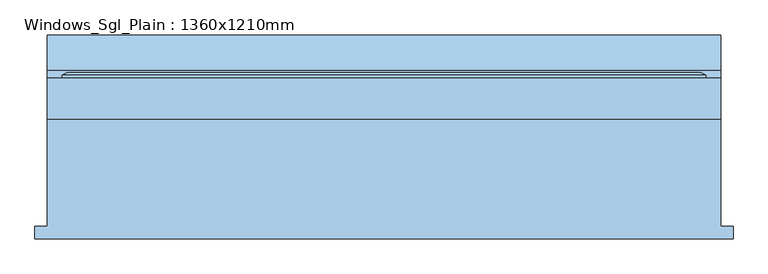
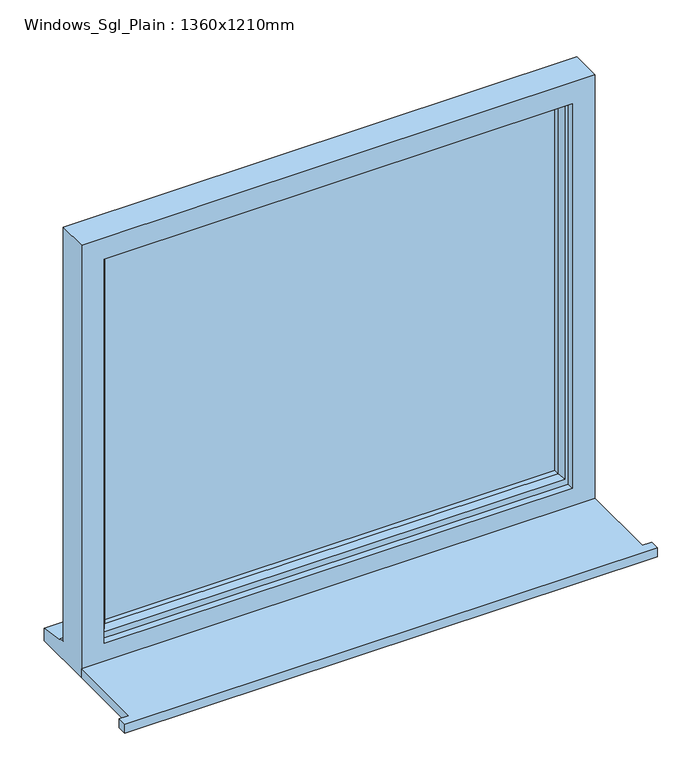
"""IFC4 building model written with IfcOpenShell, lengths in millimetres: window geometry, Windows_Sgl_Plain : 1360x1210mm."""

import ifcopenshell
import ifcopenshell.guid

model = None  # the IFC model being written
_history = None  # IfcOwnerHistory: only IFC2X3 demands one
_inside = {}  # id of a spatial element -> (the spatial element, [elements in it])
_under = {}  # id of a project, library or spatial element -> (it, [spatial elements below it])
_declared = {}  # id of a project -> (the project, [libraries it declares])
_typed = {}  # id of a type object -> (the type object, [elements of that type])
_made_of = {}  # id of a material, layer set ... -> (it, [elements and type objects made of it])


def new_model(schema):
    """Start an empty IFC model of exactly this schema.

    Asked for "IFC4X3", IfcOpenShell would pick the latest addendum, in which some entities
    have other attributes; the version numbers below select the first issue.
    IFC2X3 requires an IfcOwnerHistory on every rooted entity: one is made here for all.
    """
    global model, _history
    if schema == "IFC4X3":
        model = ifcopenshell.file(schema_version=(4, 3, 0, 0))
    else:
        model = ifcopenshell.file(schema=schema)
    _inside.clear()
    _under.clear()
    _declared.clear()
    _typed.clear()
    _made_of.clear()
    _history = None
    if model.schema == "IFC2X3":
        org = make("IfcOrganization", Name="unknown")
        user = make(
            "IfcPersonAndOrganization",
            ThePerson=make("IfcPerson", FamilyName="unknown"),
            TheOrganization=org,
        )
        app = make(
            "IfcApplication",
            ApplicationDeveloper=org,
            Version="unknown",
            ApplicationFullName="unknown",
            ApplicationIdentifier="unknown",
        )
        _history = make(
            "IfcOwnerHistory",
            OwningUser=user,
            OwningApplication=app,
            ChangeAction="ADDED",
            CreationDate=0,
        )
    return model


def make(cls, **values):
    """One entity of the class cls with the attributes given. An attribute that is None is left unset."""
    return model.create_entity(
        cls, **{name: value for name, value in values.items() if value is not None}
    )


def rooted(cls, **values):
    """An entity with a GlobalId (a new one), such as an element, a storey or a relation."""
    return make(cls, GlobalId=ifcopenshell.guid.new(), OwnerHistory=_history, **values)


def si_unit(unit_type, name, prefix=None):
    """IfcSIUnit, for example si_unit("LENGTHUNIT", "METRE", prefix="MILLI")."""
    return make("IfcSIUnit", UnitType=unit_type, Prefix=prefix, Name=name)


def assignment(units):
    """IfcUnitAssignment: the units of a project."""
    return None if units is None else make("IfcUnitAssignment", Units=units)


def point(xyz):
    """IfcCartesianPoint."""
    return None if xyz is None else make("IfcCartesianPoint", Coordinates=xyz)


def direction(xyz):
    """IfcDirection."""
    return None if xyz is None else make("IfcDirection", DirectionRatios=xyz)


def frame(location, z_axis=None, x_axis=None):
    """IfcAxis2Placement3D, a coordinate frame: its origin and axes. An axis left out is left unset."""
    return make(
        "IfcAxis2Placement3D",
        Location=point(location),
        Axis=direction(z_axis),
        RefDirection=direction(x_axis),
    )


def origin():
    """The frame at (0, 0, 0) with its axes left unset."""
    return frame((0.0, 0.0, 0.0))


def place(relative_to, where):
    """IfcLocalPlacement: puts the frame where relative to a parent placement (None: the world)."""
    return make(
        "IfcLocalPlacement", PlacementRelTo=relative_to, RelativePlacement=where
    )


def context(
    kind, dimensions, precision=None, world=None, true_north=None, identifier=None
):
    """IfcGeometricRepresentationContext, for example the 3D "Model" context."""
    return make(
        "IfcGeometricRepresentationContext",
        ContextIdentifier=identifier,
        ContextType=kind,
        CoordinateSpaceDimension=dimensions,
        Precision=precision,
        WorldCoordinateSystem=world,
        TrueNorth=true_north,
    )


def project(units=None, contexts=None):
    """IfcProject with its units and contexts."""
    return rooted(
        "IfcProject",
        Name="project",
        RepresentationContexts=contexts,
        UnitsInContext=assignment(units),
    )


def spatial(cls, under=None, at=None, **own):
    """A site, building, storey or space (cls), placed at a placement, below another one or the project."""
    s = rooted(cls, ObjectPlacement=at, **own)
    if under is not None:
        _under.setdefault(under.id(), (under, []))[1].append(s)
    return s


def polyline(points):
    """IfcPolyline through the points."""
    return make("IfcPolyline", Points=[point(p) for p in points])


def outline(outer, holes=None, kind="AREA"):
    """IfcArbitraryClosedProfileDef: a profile drawn as a closed curve; with holes, ...WithVoids."""
    if holes is None:
        return make("IfcArbitraryClosedProfileDef", ProfileType=kind, OuterCurve=outer)
    return make(
        "IfcArbitraryProfileDefWithVoids",
        ProfileType=kind,
        OuterCurve=outer,
        InnerCurves=holes,
    )


def extrude(swept, where, along, depth):
    """IfcExtrudedAreaSolid: the profile swept, set in the frame where, extruded along a direction by depth."""
    return make(
        "IfcExtrudedAreaSolid",
        SweptArea=swept,
        Position=where,
        ExtrudedDirection=direction(along),
        Depth=depth,
    )


def faces_of(points, faces, orient=None, outer=None):
    """IfcFace entities. A face is a list of loops; a loop is a list of indices into points, from 0.

    orient and outer hold one flag for each loop. By default every Orientation is true, the
    first loop of a face is its IfcFaceOuterBound and the others are IfcFaceBound.
    """
    made = []
    for i, loops in enumerate(faces):
        bounds = []
        for j, loop in enumerate(loops):
            is_outer = j == 0 if outer is None else outer[i][j]
            bounds.append(
                make(
                    "IfcFaceOuterBound" if is_outer else "IfcFaceBound",
                    Bound=make("IfcPolyLoop", Polygon=[points[k] for k in loop]),
                    Orientation=True if orient is None else orient[i][j],
                )
            )
        made.append(make("IfcFace", Bounds=bounds))
    return made


def faceted_brep(points, faces, orient=None, outer=None, voids=None):
    """IfcFacetedBrep: a solid bounded by flat faces; with voids (closed shells), ...WithVoids."""
    shared = [point(p) for p in points]
    hull = make("IfcClosedShell", CfsFaces=faces_of(shared, faces, orient, outer))
    if voids is None:
        return make("IfcFacetedBrep", Outer=hull)
    return make(
        "IfcFacetedBrepWithVoids",
        Outer=hull,
        Voids=[
            make(cls, CfsFaces=faces_of(shared, fs, o, b)) for cls, fs, o, b in voids
        ],
    )


def shape(context_of_items, identifier, shape_type, items):
    """IfcShapeRepresentation: the items that make up one representation, for example the "Body"."""
    return make(
        "IfcShapeRepresentation",
        ContextOfItems=context_of_items,
        RepresentationIdentifier=identifier,
        RepresentationType=shape_type,
        Items=items,
    )


def source(mapping_origin, context_of_items, identifier, shape_type, items):
    """IfcRepresentationMap: a shape defined once, which mapped items show again and again."""
    return make(
        "IfcRepresentationMap",
        MappingOrigin=mapping_origin,
        MappedRepresentation=shape(context_of_items, identifier, shape_type, items),
    )


def transform(
    local_origin,
    x_axis=None,
    y_axis=None,
    z_axis=None,
    scale=None,
    scale2=None,
    scale3=None,
    uniform=True,
):
    """IfcCartesianTransformationOperator3D, or its non-uniform kind. x_axis, y_axis, z_axis: its Axis1, 2, 3."""
    if uniform:
        return make(
            "IfcCartesianTransformationOperator3D",
            Axis1=direction(x_axis),
            Axis2=direction(y_axis),
            LocalOrigin=point(local_origin),
            Scale=scale,
            Axis3=direction(z_axis),
        )
    return make(
        "IfcCartesianTransformationOperator3DnonUniform",
        Axis1=direction(x_axis),
        Axis2=direction(y_axis),
        LocalOrigin=point(local_origin),
        Scale=scale,
        Axis3=direction(z_axis),
        Scale2=scale2,
        Scale3=scale3,
    )


def mapped(mapping_source, mapping_target):
    """IfcMappedItem: shows the shape of a source again, moved by a transform."""
    return make(
        "IfcMappedItem", MappingSource=mapping_source, MappingTarget=mapping_target
    )


def made_of(thing, what):
    """Note that an element or type object is made of a material, layer set ...; save() writes the relation."""
    if what is not None:
        _made_of.setdefault(what.id(), (what, []))[1].append(thing)
    return thing


def element(
    cls,
    number,
    at=None,
    inside=None,
    cuts=None,
    type_object=None,
    material=None,
    context=None,
    identifier="Body",
    shape_type=None,
    held_by="IfcProductDefinitionShape",
    body=None,
    shapes=None,
    **own,
):
    """One element of the class cls, such as IfcWall. Its Tag is "e" and its number.

    at: its placement. inside: the storey or other place that contains it. cuts: it is an
    opening in that element (IfcRelVoidsElement). A single representation is given by context,
    identifier, shape_type and body (its items); several are given by shapes. held_by: the class
    of the entity that holds the representations. save() writes the other relations.
    """
    e = rooted(cls, Tag="e%d" % number, ObjectPlacement=at, **own)
    if body is not None:
        shapes = [shape(context, identifier, shape_type, body)]
    if shapes is not None:
        e.Representation = make(held_by, Representations=shapes)
    if inside is not None:
        _inside.setdefault(inside.id(), (inside, []))[1].append(e)
    if cuts is not None:
        rooted(
            "IfcRelVoidsElement", RelatingBuildingElement=cuts, RelatedOpeningElement=e
        )
    if type_object is not None:
        _typed.setdefault(type_object.id(), (type_object, []))[1].append(e)
    return made_of(e, material)


def aggregate(whole, parts):
    """IfcRelAggregates: a whole, such as a stair, and the parts it consists of."""
    return rooted("IfcRelAggregates", RelatingObject=whole, RelatedObjects=parts)


def save(model, path):
    """Write the relations noted so far, then the file.

    IfcRelAggregates (storeys below a building ...), IfcRelContainedInSpatialStructure (elements
    in a storey), IfcRelDefinesByType, IfcRelAssociatesMaterial and IfcRelDeclares: one each for
    every whole, place, type object, material and project.
    """
    for whole, parts in _under.values():
        aggregate(whole, parts)
    for where, things in _inside.values():
        rooted(
            "IfcRelContainedInSpatialStructure",
            RelatedElements=things,
            RelatingStructure=where,
        )
    for kind, things in _typed.values():
        rooted("IfcRelDefinesByType", RelatedObjects=things, RelatingType=kind)
    for what, things in _made_of.values():
        rooted("IfcRelAssociatesMaterial", RelatedObjects=things, RelatingMaterial=what)
    for by, libraries in _declared.values():
        rooted("IfcRelDeclares", RelatingContext=by, RelatedDefinitions=libraries)
    model.write(path)


def windows_sgl_plain_1360x1210mm_bb3badfb(model_context):
    return source(origin(), model_context, "Body", "SolidModel", [
        extrude(outline(polyline([(-705.0, -191.5434322), (-705.0, -166.5434322), (-680.0, -166.5434322), (-680.0, 50.4565678), (680.0, 50.4565678), (680.0, -166.5434322), (705.0, -166.5434322), (705.0, -191.5434322), (-705.0, -191.5434322)])), frame((0.0, 0.0, 900.0), z_axis=(0.0, 0.0, 1.0), x_axis=(1.0, 0.0, 0.0)), (0.0, 0.0, 1.0), 25.0),
        faceted_brep([(-680.0, 50.4565678, 900.0), (680.0, 50.4565678, 900.0), (680.0, 50.4565678, 2110.0), (-680.0, 50.4565678, 2110.0), (-620.0, 50.4565678, 2050.0), (620.0, 50.4565678, 2050.0), (620.0, 50.4565678, 975.0), (-620.0, 50.4565678, 975.0), (-680.0, 133.4565678, 2110.0), (-680.0, 133.4565678, 951.0), (-680.0, 148.4565678, 949.68767), (-680.0, 148.4565678, 944.7449676), (-680.0, 220.9565678, 933.8088847), (-680.0, 220.9565678, 900.0), (680.0, 133.4565678, 2110.0), (680.0, 133.4565678, 951.0), (-640.0, 133.4565678, 2070.0), (-640.0, 133.4565678, 963.0), (640.0, 133.4565678, 963.0), (640.0, 133.4565678, 2070.0), (-640.0, 68.4565678, 2070.0), (-640.0, 68.4565678, 963.0), (640.0, 68.4565678, 2070.0), (640.0, 68.4565678, 963.0), (-620.0, 68.4565678, 2050.0), (-620.0, 68.4565678, 975.0), (620.0, 68.4565678, 975.0), (620.0, 68.4565678, 2050.0), (680.0, 220.9565678, 900.0), (680.0, 220.9565678, 933.8088847), (680.0, 148.4565678, 944.7449676), (680.0, 148.4565678, 949.68767)], [[[0, 1, 2, 3], [4, 5, 6, 7]], [[0, 3, 8, 9, 10, 11, 12, 13]], [[9, 8, 14, 15], [16, 17, 18, 19]], [[17, 16, 20, 21]], [[20, 22, 23, 21], [24, 25, 26, 27]], [[24, 4, 7, 25]], [[3, 2, 14, 8]], [[16, 19, 22, 20]], [[5, 4, 24, 27]], [[15, 14, 2, 1, 28, 29, 30, 31]], [[19, 18, 23, 22]], [[5, 27, 26, 6]], [[28, 1, 0, 13]], [[29, 28, 13, 12]], [[30, 29, 12, 11]], [[31, 30, 11, 10]], [[15, 31, 10, 9]], [[21, 23, 18, 17]], [[7, 6, 26, 25]]]),
        extrude(outline(polyline([(610.0, 97.4565678), (-610.0, 97.4565678), (-610.0, 121.4565678), (610.0, 121.4565678), (610.0, 97.4565678)])), frame((0.0, 0.0, 993.0), z_axis=(0.0, 0.0, 1.0), x_axis=(1.0, 0.0, 0.0)), (0.0, 0.0, 1.0), 1047.0),
        faceted_brep([(-650.0, 133.4565678, 2080.0), (-650.0, 139.2300705, 2080.0), (-650.0, 139.2300705, 953.0), (-650.0, 133.4565678, 953.0), (-640.0, 68.4565678, 2070.0), (-640.0, 133.4565678, 2070.0), (-640.0, 133.4565678, 963.0), (-640.0, 68.4565678, 963.0), (-600.0, 82.9494677, 2030.0), (-610.1480377, 68.4565678, 2040.1480377), (-610.1480377, 68.4565678, 992.8519623), (-600.0, 82.9494677, 1003.0), (-600.0, 97.4565678, 2030.0), (-600.0, 97.4565678, 1003.0), (-610.0, 121.4565678, 2040.0), (-610.0, 97.4565678, 2040.0), (-610.0, 97.4565678, 993.0), (-610.0, 121.4565678, 993.0), (-600.0, 139.2300705, 2030.0), (-600.0, 121.4565678, 2030.0), (-600.0, 121.4565678, 1003.0), (-600.0, 139.2300705, 1003.0), (-617.4457548, 145.0035732, 2047.4457548), (-617.4457548, 145.0035732, 985.5542452), (-639.2153903, 145.0035732, 2069.2153903), (-639.2153903, 145.0035732, 963.7846097), (650.0, 139.2300705, 953.0), (650.0, 133.4565678, 953.0), (640.0, 133.4565678, 963.0), (640.0, 68.4565678, 963.0), (610.1480377, 68.4565678, 992.8519623), (600.0, 82.9494677, 1003.0), (600.0, 97.4565678, 1003.0), (610.0, 97.4565678, 993.0), (610.0, 121.4565678, 993.0), (600.0, 121.4565678, 1003.0), (600.0, 139.2300705, 1003.0), (617.4457548, 145.0035732, 985.5542452), (639.2153903, 145.0035732, 963.7846097), (650.0, 139.2300705, 2080.0), (650.0, 133.4565678, 2080.0), (640.0, 133.4565678, 2070.0), (640.0, 68.4565678, 2070.0), (610.1480377, 68.4565678, 2040.1480377), (600.0, 82.9494677, 2030.0), (600.0, 97.4565678, 2030.0), (610.0, 97.4565678, 2040.0), (610.0, 121.4565678, 2040.0), (600.0, 121.4565678, 2030.0), (600.0, 139.2300705, 2030.0), (617.4457548, 145.0035732, 2047.4457548), (639.2153903, 145.0035732, 2069.2153903)], [[[0, 1, 2, 3]], [[4, 5, 6, 7]], [[8, 9, 10, 11]], [[12, 8, 11, 13]], [[14, 15, 16, 17]], [[18, 19, 20, 21]], [[22, 18, 21, 23]], [[1, 24, 25, 2]], [[3, 2, 26, 27]], [[7, 6, 28, 29]], [[11, 10, 30, 31]], [[13, 11, 31, 32]], [[17, 16, 33, 34]], [[21, 20, 35, 36]], [[23, 21, 36, 37]], [[2, 25, 38, 26]], [[27, 26, 39, 40]], [[29, 28, 41, 42]], [[31, 30, 43, 44]], [[32, 31, 44, 45]], [[34, 33, 46, 47]], [[36, 35, 48, 49]], [[37, 36, 49, 50]], [[26, 38, 51, 39]], [[40, 39, 1, 0]], [[3, 27, 40, 0], [5, 41, 28, 6]], [[42, 41, 5, 4]], [[7, 29, 42, 4], [9, 43, 30, 10]], [[44, 43, 9, 8]], [[45, 44, 8, 12]], [[15, 46, 33, 16], [13, 32, 45, 12]], [[47, 46, 15, 14]], [[17, 34, 47, 14], [19, 48, 35, 20]], [[49, 48, 19, 18]], [[50, 49, 18, 22]], [[24, 51, 38, 25], [23, 37, 50, 22]], [[39, 51, 24, 1]]]),
    ])


if __name__ == "__main__":
    model = new_model("IFC4")
    model_context = context("Model", 3, world=origin())
    ifc_project = project(units=[si_unit("LENGTHUNIT", "METRE", prefix="MILLI")], contexts=[model_context])
    site = spatial("IfcSite", under=ifc_project)
    building = spatial("IfcBuilding", under=site)
    placement = place(None, origin())
    windows_sgl_plain_1360x1210mm_shape = windows_sgl_plain_1360x1210mm_bb3badfb(model_context)
    element("IfcWindow", 1, ObjectType="Windows_Sgl_Plain : 1360x1210mm", at=placement, inside=building, context=model_context, shape_type="MappedRepresentation", body=[
        mapped(windows_sgl_plain_1360x1210mm_shape, transform((0.0, 0.0, 0.0), x_axis=(1.0, 0.0, 0.0), y_axis=(0.0, 1.0, 0.0), z_axis=(0.0, 0.0, 1.0))),
    ])
    save(model, "model.ifc")

# Revit data of these elements
# Type "Windows_Sgl_Plain : 1360x1210mm"
#   Type Mark = "47"
#   Operation = "SinglePanel"
#   Construction Type Id = "SGL"
#   Manufacturer = "Revit"
#   Keynote = "L10"
#   Analytic Construction = "Large single-glazed windows"
#   Wrap Layers (Ext) from Ext = 102.5 mm
#   Wrap Layers (Int) from Ext = 177.5 mm
#   Window Board Projection = 25 mm
#   Window Board Extension = 25 mm
#   Visual Light Transmittance = 0.9
#   Solar Heat Gain Coefficient = 0.86
#   Rough Width = 1360 mm
#   Rough Height = 1210 mm
#   Height = 1210 mm
#   Width = 1360 mm
#   Heat Transfer Coefficient (U) = 5.5617 W/(m²·K)
#   Glazing Thickness = 24 mm
#   FrameOffset - External = 50 mm
#   Frame Depth = 65 mm
#   Default Head Height = 2110 mm
#   Cill Depth = 87.5 mm
#   Cavity Closer Width = 50 mm
#   Cavity Closer Offset from Ext = 102.5 mm
#   Cavity Closer Depth = 85 mm
#   Vis - Cavity Closers = yes
#   Define Thermal Properties by = 1
#   Material Trim = Window Frame
#   Material Glass = Glass
#   Material Frame = Window Frame
#   Wall Closure = (empty or 0)
# Element 1 (IfcWindow, "Windows_Sgl_Plain : 1360x1210mm")
#   Materials on its faces: "Window Frame", "Glass"
# Materials
#   "Window Frame": class "Miscellaneous", colour RGB 249 249 249, transparency 0, Keynote = "L10", Cost = 0
#   "Glass": class "Glass", colour RGB 0 128 192, transparency 0.9, Description = "Soda Lime Glass", Cost = 0
